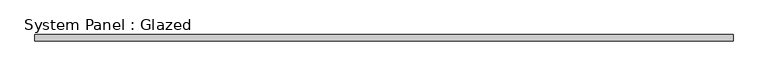
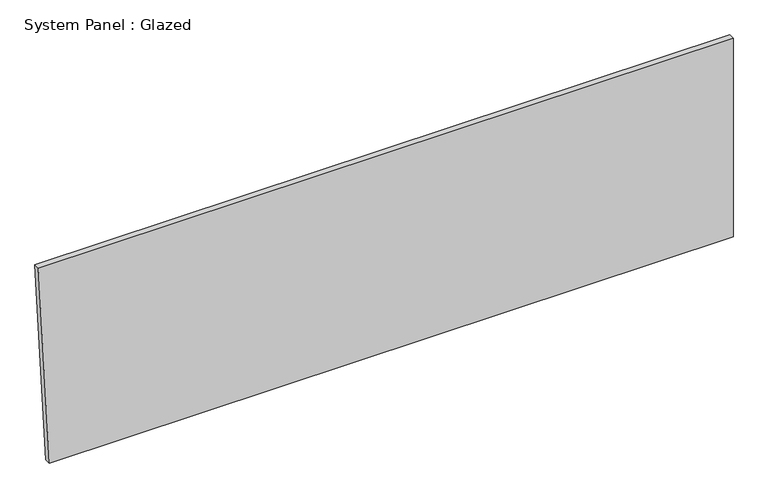
"""IFC4 building model written with IfcOpenShell, lengths in millimetres: plate geometry, System Panel : Glazed."""

import ifcopenshell
import ifcopenshell.guid

model = None  # the IFC model being written
_history = None  # IfcOwnerHistory: only IFC2X3 demands one
_inside = {}  # id of a spatial element -> (the spatial element, [elements in it])
_under = {}  # id of a project, library or spatial element -> (it, [spatial elements below it])
_declared = {}  # id of a project -> (the project, [libraries it declares])
_typed = {}  # id of a type object -> (the type object, [elements of that type])
_made_of = {}  # id of a material, layer set ... -> (it, [elements and type objects made of it])


def new_model(schema):
    """Start an empty IFC model of exactly this schema.

    Asked for "IFC4X3", IfcOpenShell would pick the latest addendum, in which some entities
    have other attributes; the version numbers below select the first issue.
    IFC2X3 requires an IfcOwnerHistory on every rooted entity: one is made here for all.
    """
    global model, _history
    if schema == "IFC4X3":
        model = ifcopenshell.file(schema_version=(4, 3, 0, 0))
    else:
        model = ifcopenshell.file(schema=schema)
    _inside.clear()
    _under.clear()
    _declared.clear()
    _typed.clear()
    _made_of.clear()
    _history = None
    if model.schema == "IFC2X3":
        org = make("IfcOrganization", Name="unknown")
        user = make(
            "IfcPersonAndOrganization",
            ThePerson=make("IfcPerson", FamilyName="unknown"),
            TheOrganization=org,
        )
        app = make(
            "IfcApplication",
            ApplicationDeveloper=org,
            Version="unknown",
            ApplicationFullName="unknown",
            ApplicationIdentifier="unknown",
        )
        _history = make(
            "IfcOwnerHistory",
            OwningUser=user,
            OwningApplication=app,
            ChangeAction="ADDED",
            CreationDate=0,
        )
    return model


def make(cls, **values):
    """One entity of the class cls with the attributes given. An attribute that is None is left unset."""
    return model.create_entity(
        cls, **{name: value for name, value in values.items() if value is not None}
    )


def rooted(cls, **values):
    """An entity with a GlobalId (a new one), such as an element, a storey or a relation."""
    return make(cls, GlobalId=ifcopenshell.guid.new(), OwnerHistory=_history, **values)


def si_unit(unit_type, name, prefix=None):
    """IfcSIUnit, for example si_unit("LENGTHUNIT", "METRE", prefix="MILLI")."""
    return make("IfcSIUnit", UnitType=unit_type, Prefix=prefix, Name=name)


def assignment(units):
    """IfcUnitAssignment: the units of a project."""
    return None if units is None else make("IfcUnitAssignment", Units=units)


def point(xyz):
    """IfcCartesianPoint."""
    return None if xyz is None else make("IfcCartesianPoint", Coordinates=xyz)


def direction(xyz):
    """IfcDirection."""
    return None if xyz is None else make("IfcDirection", DirectionRatios=xyz)


def frame(location, z_axis=None, x_axis=None):
    """IfcAxis2Placement3D, a coordinate frame: its origin and axes. An axis left out is left unset."""
    return make(
        "IfcAxis2Placement3D",
        Location=point(location),
        Axis=direction(z_axis),
        RefDirection=direction(x_axis),
    )


def origin():
    """The frame at (0, 0, 0) with its axes left unset."""
    return frame((0.0, 0.0, 0.0))


def place(relative_to, where):
    """IfcLocalPlacement: puts the frame where relative to a parent placement (None: the world)."""
    return make(
        "IfcLocalPlacement", PlacementRelTo=relative_to, RelativePlacement=where
    )


def context(
    kind, dimensions, precision=None, world=None, true_north=None, identifier=None
):
    """IfcGeometricRepresentationContext, for example the 3D "Model" context."""
    return make(
        "IfcGeometricRepresentationContext",
        ContextIdentifier=identifier,
        ContextType=kind,
        CoordinateSpaceDimension=dimensions,
        Precision=precision,
        WorldCoordinateSystem=world,
        TrueNorth=true_north,
    )


def project(units=None, contexts=None):
    """IfcProject with its units and contexts."""
    return rooted(
        "IfcProject",
        Name="project",
        RepresentationContexts=contexts,
        UnitsInContext=assignment(units),
    )


def spatial(cls, under=None, at=None, **own):
    """A site, building, storey or space (cls), placed at a placement, below another one or the project."""
    s = rooted(cls, ObjectPlacement=at, **own)
    if under is not None:
        _under.setdefault(under.id(), (under, []))[1].append(s)
    return s


def polyline(points):
    """IfcPolyline through the points."""
    return make("IfcPolyline", Points=[point(p) for p in points])


def outline(outer, holes=None, kind="AREA"):
    """IfcArbitraryClosedProfileDef: a profile drawn as a closed curve; with holes, ...WithVoids."""
    if holes is None:
        return make("IfcArbitraryClosedProfileDef", ProfileType=kind, OuterCurve=outer)
    return make(
        "IfcArbitraryProfileDefWithVoids",
        ProfileType=kind,
        OuterCurve=outer,
        InnerCurves=holes,
    )


def extrude(swept, where, along, depth):
    """IfcExtrudedAreaSolid: the profile swept, set in the frame where, extruded along a direction by depth."""
    return make(
        "IfcExtrudedAreaSolid",
        SweptArea=swept,
        Position=where,
        ExtrudedDirection=direction(along),
        Depth=depth,
    )


def shape(context_of_items, identifier, shape_type, items):
    """IfcShapeRepresentation: the items that make up one representation, for example the "Body"."""
    return make(
        "IfcShapeRepresentation",
        ContextOfItems=context_of_items,
        RepresentationIdentifier=identifier,
        RepresentationType=shape_type,
        Items=items,
    )


def source(mapping_origin, context_of_items, identifier, shape_type, items):
    """IfcRepresentationMap: a shape defined once, which mapped items show again and again."""
    return make(
        "IfcRepresentationMap",
        MappingOrigin=mapping_origin,
        MappedRepresentation=shape(context_of_items, identifier, shape_type, items),
    )


def transform(
    local_origin,
    x_axis=None,
    y_axis=None,
    z_axis=None,
    scale=None,
    scale2=None,
    scale3=None,
    uniform=True,
):
    """IfcCartesianTransformationOperator3D, or its non-uniform kind. x_axis, y_axis, z_axis: its Axis1, 2, 3."""
    if uniform:
        return make(
            "IfcCartesianTransformationOperator3D",
            Axis1=direction(x_axis),
            Axis2=direction(y_axis),
            LocalOrigin=point(local_origin),
            Scale=scale,
            Axis3=direction(z_axis),
        )
    return make(
        "IfcCartesianTransformationOperator3DnonUniform",
        Axis1=direction(x_axis),
        Axis2=direction(y_axis),
        LocalOrigin=point(local_origin),
        Scale=scale,
        Axis3=direction(z_axis),
        Scale2=scale2,
        Scale3=scale3,
    )


def mapped(mapping_source, mapping_target):
    """IfcMappedItem: shows the shape of a source again, moved by a transform."""
    return make(
        "IfcMappedItem", MappingSource=mapping_source, MappingTarget=mapping_target
    )


def made_of(thing, what):
    """Note that an element or type object is made of a material, layer set ...; save() writes the relation."""
    if what is not None:
        _made_of.setdefault(what.id(), (what, []))[1].append(thing)
    return thing


def element(
    cls,
    number,
    at=None,
    inside=None,
    cuts=None,
    type_object=None,
    material=None,
    context=None,
    identifier="Body",
    shape_type=None,
    held_by="IfcProductDefinitionShape",
    body=None,
    shapes=None,
    **own,
):
    """One element of the class cls, such as IfcWall. Its Tag is "e" and its number.

    at: its placement. inside: the storey or other place that contains it. cuts: it is an
    opening in that element (IfcRelVoidsElement). A single representation is given by context,
    identifier, shape_type and body (its items); several are given by shapes. held_by: the class
    of the entity that holds the representations. save() writes the other relations.
    """
    e = rooted(cls, Tag="e%d" % number, ObjectPlacement=at, **own)
    if body is not None:
        shapes = [shape(context, identifier, shape_type, body)]
    if shapes is not None:
        e.Representation = make(held_by, Representations=shapes)
    if inside is not None:
        _inside.setdefault(inside.id(), (inside, []))[1].append(e)
    if cuts is not None:
        rooted(
            "IfcRelVoidsElement", RelatingBuildingElement=cuts, RelatedOpeningElement=e
        )
    if type_object is not None:
        _typed.setdefault(type_object.id(), (type_object, []))[1].append(e)
    return made_of(e, material)


def aggregate(whole, parts):
    """IfcRelAggregates: a whole, such as a stair, and the parts it consists of."""
    return rooted("IfcRelAggregates", RelatingObject=whole, RelatedObjects=parts)


def save(model, path):
    """Write the relations noted so far, then the file.

    IfcRelAggregates (storeys below a building ...), IfcRelContainedInSpatialStructure (elements
    in a storey), IfcRelDefinesByType, IfcRelAssociatesMaterial and IfcRelDeclares: one each for
    every whole, place, type object, material and project.
    """
    for whole, parts in _under.values():
        aggregate(whole, parts)
    for where, things in _inside.values():
        rooted(
            "IfcRelContainedInSpatialStructure",
            RelatedElements=things,
            RelatingStructure=where,
        )
    for kind, things in _typed.values():
        rooted("IfcRelDefinesByType", RelatedObjects=things, RelatingType=kind)
    for what, things in _made_of.values():
        rooted("IfcRelAssociatesMaterial", RelatedObjects=things, RelatingMaterial=what)
    for by, libraries in _declared.values():
        rooted("IfcRelDeclares", RelatingContext=by, RelatedDefinitions=libraries)
    model.write(path)


def system_panel_glazed_b0ec51c6(model_context):
    return source(origin(), model_context, "Body", "SweptSolid", [
        extrude(outline(polyline([(0.0, -1389.0768125), (0.0, 1434.3998477), (866.0018549, 1434.3998477), (866.0018549, -1434.3998477), (0.0, -1389.0768125)])), frame((0.0, -44.45, 0.0), z_axis=(0.0, 1.0, 0.0), x_axis=(0.0, 0.0, 1.0)), (0.0, 0.0, 1.0), 25.4),
    ])


if __name__ == "__main__":
    model = new_model("IFC4")
    model_context = context("Model", 3, world=origin())
    ifc_project = project(units=[si_unit("LENGTHUNIT", "METRE", prefix="MILLI")], contexts=[model_context])
    site = spatial("IfcSite", under=ifc_project)
    building = spatial("IfcBuilding", under=site)
    placement = place(None, origin())
    system_panel_glazed_shape = system_panel_glazed_b0ec51c6(model_context)
    element("IfcPlate", 1, ObjectType="System Panel : Glazed", at=placement, inside=building, context=model_context, shape_type="MappedRepresentation", body=[
        mapped(system_panel_glazed_shape, transform((0.0, 0.0, 0.0), x_axis=(1.0, 0.0, 0.0), y_axis=(0.0, 1.0, 0.0), z_axis=(0.0, 0.0, 1.0))),
    ])
    save(model, "model.ifc")

# Revit data of these elements
# Type "System Panel : Glazed"
#   Construction Type Id = "GSP4R"
#   Analytic Construction = "1/8 in Pilkington single glazing"
#   Visual Light Transmittance = 0.9
#   Solar Heat Gain Coefficient = 0.86
#   Heat Transfer Coefficient (U) = 1.18115 BTU/(h·ft²·°F)
#   Define Thermal Properties by = 1
# Element 1 (IfcPlate, "System Panel : Glazed")
#   Materials on its faces: "Glass"
# Materials
#   "Glass": class "Glass", colour RGB 0 128 192, transparency 0.75, Description = "Soda Lime Glass", Cost = 0
